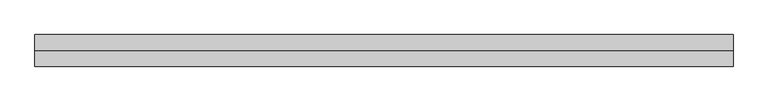
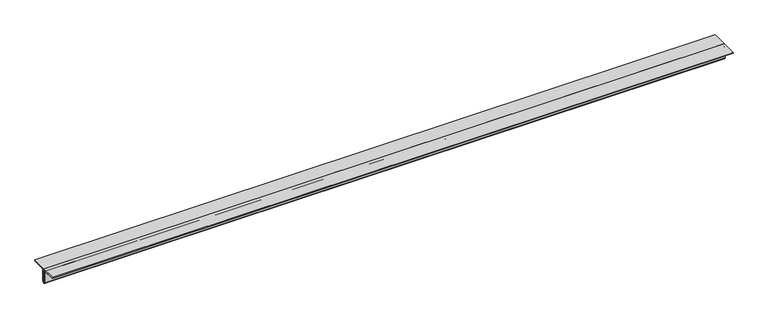
"""IFC4 building model written with IfcOpenShell, lengths in millimetres: member geometry, 0123_Steel Framing_2Ls-KSD3502 : H_SB_AR_S03_2Ls-130x130x12_HBR4."""

from ifc_helpers import new_model, si_unit, point, frame, frame_2d, origin, place, context, project, spatial, polyline, circle_curve, trimmed, segment, composite_curve, outline, extrude, source, transform, mapped, element, save


def member_d5462e7f(model_context):
    return source(origin(), model_context, "Body", "SweptSolid", [
        extrude(outline(composite_curve([segment(polyline([(0.0, 36.4), (130.0, 36.4)]), True, "CONTINUOUS"), segment(trimmed(circle_curve(frame_2d((118.0, 36.4)), 12.0), [point((130.0, 36.4))], [point((118.0, 24.4))], False, "CARTESIAN"), True, "CONTINUOUS"), segment(polyline([(118.0, 24.4), (24.0, 24.4)]), True, "CONTINUOUS"), segment(trimmed(circle_curve(frame_2d((24.0, 12.4)), 12.0), [point((24.0, 24.4))], [point((12.0, 12.4))], True, "CARTESIAN"), True, "CONTINUOUS"), segment(polyline([(12.0, 12.4), (12.0, -81.6)]), True, "CONTINUOUS"), segment(trimmed(circle_curve(frame_2d((0.0, -81.6)), 12.0), [point((12.0, -81.6))], [point((0.0, -93.6))], False, "CARTESIAN"), True, "CONTINUOUS"), segment(polyline([(0.0, -93.6), (0.0, 36.4)]), True, "CONTINUOUS")], self_intersect=False)), frame((-2800.6519893, 0.0, 0.0), z_axis=(1.0, 0.0, 0.0), x_axis=(0.0, 1.0, 0.0)), (0.0, 0.0, 1.0), 5733.5453123),
        extrude(outline(composite_curve([segment(polyline([(0.0, 36.4), (0.0, -93.6)]), True, "CONTINUOUS"), segment(trimmed(circle_curve(frame_2d((0.0, -81.6)), 12.0), [point((0.0, -93.6))], [point((-12.0, -81.6))], False, "CARTESIAN"), True, "CONTINUOUS"), segment(polyline([(-12.0, -81.6), (-12.0, 12.4)]), True, "CONTINUOUS"), segment(trimmed(circle_curve(frame_2d((-24.0, 12.4)), 12.0), [point((-12.0, 12.4))], [point((-24.0, 24.4))], True, "CARTESIAN"), True, "CONTINUOUS"), segment(polyline([(-24.0, 24.4), (-118.0, 24.4)]), True, "CONTINUOUS"), segment(trimmed(circle_curve(frame_2d((-118.0, 36.4)), 12.0), [point((-118.0, 24.4))], [point((-130.0, 36.4))], False, "CARTESIAN"), True, "CONTINUOUS"), segment(polyline([(-130.0, 36.4), (0.0, 36.4)]), True, "CONTINUOUS")], self_intersect=False)), frame((-2800.6519893, 0.0, 0.0), z_axis=(1.0, 0.0, 0.0), x_axis=(0.0, 1.0, 0.0)), (0.0, 0.0, 1.0), 5733.5453123),
    ])


if __name__ == "__main__":
    model = new_model("IFC4")
    model_context = context("Model", 3, world=origin())
    ifc_project = project(units=[si_unit("LENGTHUNIT", "METRE", prefix="MILLI")], contexts=[model_context])
    site = spatial("IfcSite", under=ifc_project)
    building = spatial("IfcBuilding", under=site)
    placement = place(None, origin())
    member_shape = member_d5462e7f(model_context)
    element("IfcMember", 1, ObjectType="0123_Steel Framing_2Ls-KSD3502 : H_SB_AR_S03_2Ls-130x130x12_HBR4", at=placement, inside=building, context=model_context, shape_type="MappedRepresentation", body=[
        mapped(member_shape, transform((0.0, 0.0, 0.0), x_axis=(1.0, 0.0, 0.0), y_axis=(0.0, 1.0, 0.0), z_axis=(0.0, 0.0, 1.0))),
    ])
    save(model, "model.ifc")

# Revit data of these elements
# Type "0123_Steel Framing_2Ls-KSD3502 : H_SB_AR_S03_2Ls-130x130x12_HBR4"
#   Type Mark = "HBR4"
#   Assembly Code = "B10"
#   Legs = "SLBB"
#   W = 8.97
#   Perimeter = 1.04 m²/m
#   Nominal Weight = 46.80 kgf/m
#   Length [instance default] = 1000 mm
#   Space = 0 mm
#   b = 130 mm
#   d = 130 mm
#   t = 12 mm
#   y = 36.4 mm
#   A = 0.005952 m²
#   Structural Material [instance default] = Steel ASTM A36
# Element 1 (IfcMember, "0123_Steel Framing_2Ls-KSD3502 : H_SB_AR_S03_2Ls-130x130x12_HBR4")
#   Materials on its faces: "Steel ASTM A36"
# Materials
#   "Steel ASTM A36": class "Metal", colour RGB 199 199 199, transparency 0, Description = "Structural steel, ASTM A36 Grade B, mill finish", Cost = 0
